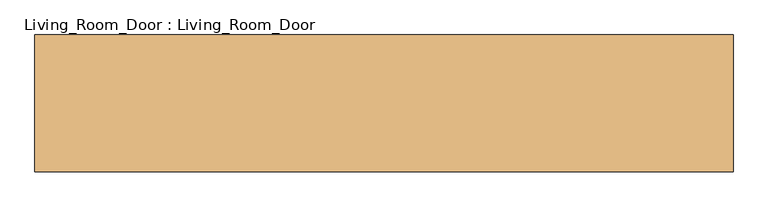
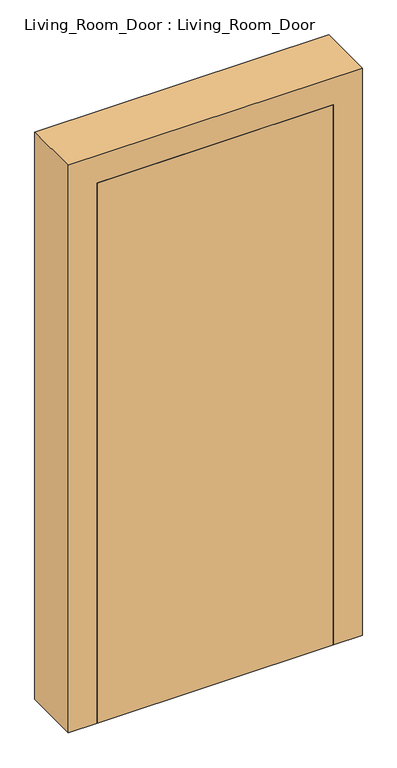
"""IFC4 building model written with IfcOpenShell, lengths in millimetres: door geometry, Living_Room_Door : Living_Room_Door."""

from ifc_helpers import new_model, si_unit, frame, origin, place, context, project, spatial, polyline, outline, extrude, source, transform, mapped, element, save


def living_room_door_living_room_door_3c1abd9c(model_context):
    return source(origin(), model_context, "Body", "SweptSolid", [
        extrude(outline(polyline([(315.0, 9545.0), (1135.0, 9545.0), (1135.0, 9445.0), (315.0, 9445.0), (315.0, 9545.0)])), frame((0.0, 0.0, 250.0), z_axis=(0.0, 0.0, 1.0), x_axis=(1.0, 0.0, 0.0)), (0.0, 0.0, 1.0), 1980.0),
        extrude(outline(polyline([(250.0, 215.0), (250.0, 315.0), (2230.0, 315.0), (2230.0, 1135.0), (250.0, 1135.0), (250.0, 1235.0), (2330.0, 1235.0), (2330.0, 215.0), (250.0, 215.0)])), frame((0.0, 9445.0, 0.0), z_axis=(0.0, 1.0, 0.0), x_axis=(0.0, 0.0, 1.0)), (0.0, 0.0, 1.0), 200.0),
    ])


if __name__ == "__main__":
    model = new_model("IFC4")
    model_context = context("Model", 3, world=origin())
    ifc_project = project(units=[si_unit("LENGTHUNIT", "METRE", prefix="MILLI")], contexts=[model_context])
    site = spatial("IfcSite", under=ifc_project)
    building = spatial("IfcBuilding", under=site)
    placement = place(None, origin())
    living_room_door_living_room_door_shape = living_room_door_living_room_door_3c1abd9c(model_context)
    element("IfcDoor", 1, ObjectType="Living_Room_Door : Living_Room_Door", at=placement, inside=building, context=model_context, shape_type="MappedRepresentation", body=[
        mapped(living_room_door_living_room_door_shape, transform((0.0, 0.0, 0.0), x_axis=(1.0, 0.0, 0.0), y_axis=(0.0, 1.0, 0.0), z_axis=(0.0, 0.0, 1.0))),
    ])
    save(model, "model.ifc")

# Revit data of these elements
# Type "Living_Room_Door : Living_Room_Door"
#   Type Mark = "51"
#   NameOverride = "Living_Room_Door"
# Element 1 (IfcDoor, "Living_Room_Door : Living_Room_Door")
#   Materials on its faces: "IfcSurfaceStyle #392"
# Materials
#   "IfcSurfaceStyle #392": class "Unassigned", colour RGB 204 204 204, transparency 0
